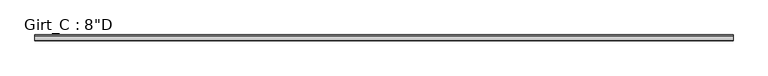
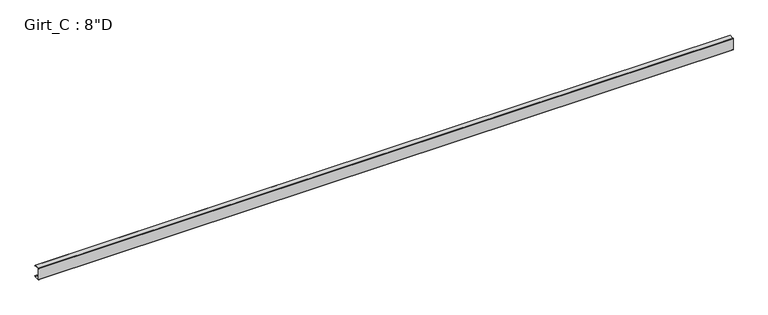
"""IFC4 building model written with IfcOpenShell, lengths in millimetres: beam geometry."""

from ifc_helpers import new_model, si_unit, point, frame, frame_2d, origin, place, context, project, spatial, polyline, circle_curve, trimmed, segment, composite_curve, outline, extrude, source, transform, mapped, element, save


def beam_9130b546(model_context):
    return source(origin(), model_context, "Body", "SweptSolid", [
        extrude(outline(composite_curve([segment(polyline([(87.5109375, 101.6), (99.7560415, 87.0068534), (97.6278742, 85.221109), (86.2154765, 98.821875), (3.3005807, 98.821875)]), True, "CONTINUOUS"), segment(trimmed(circle_curve(frame_2d((3.3741066, 96.8381931)), 1.9850441), [point((3.3005807, 98.821875))], [point((1.3890625, 96.8381931))], True, "CARTESIAN"), True, "CONTINUOUS"), segment(polyline([(1.3890625, 96.8381931), (1.3890625, -96.8389339)]), True, "CONTINUOUS"), segment(trimmed(circle_curve(frame_2d((3.3748024, -96.8389339)), 1.9857399), [point((1.3890625, -96.8389339))], [point((3.2694106, -98.821875))], True, "CARTESIAN"), True, "CONTINUOUS"), segment(polyline([(3.2694106, -98.821875), (86.2154765, -98.821875), (97.6510975, -85.1934327), (99.7792647, -86.979177), (87.5109375, -101.6), (3.3734375, -101.6)]), True, "CONTINUOUS"), segment(trimmed(circle_curve(frame_2d((3.3734375, -96.8375)), 4.7625), [point((3.3734375, -101.6))], [point((-1.3890625, -96.8375))], False, "CARTESIAN"), True, "CONTINUOUS"), segment(polyline([(-1.3890625, -96.8375), (-1.3890625, 96.8375)]), True, "CONTINUOUS"), segment(trimmed(circle_curve(frame_2d((3.3734375, 96.8375)), 4.7625), [point((-1.3890625, 96.8375))], [point((3.3734375, 101.6))], False, "CARTESIAN"), True, "CONTINUOUS"), segment(polyline([(3.3734375, 101.6), (87.5109375, 101.6)]), True, "CONTINUOUS")], self_intersect=False)), frame((-5835.65, 0.0, 0.0), z_axis=(1.0, 0.0, 0.0), x_axis=(0.0, 1.0, 0.0)), (0.0, 0.0, 1.0), 11671.3),
    ])


if __name__ == "__main__":
    model = new_model("IFC4")
    model_context = context("Model", 3, world=origin())
    ifc_project = project(units=[si_unit("LENGTHUNIT", "METRE", prefix="MILLI")], contexts=[model_context])
    site = spatial("IfcSite", under=ifc_project)
    building = spatial("IfcBuilding", under=site)
    placement = place(None, origin())
    beam_shape = beam_9130b546(model_context)
    element("IfcBeam", 1, ObjectType="Girt_C : 8\"D", at=placement, inside=building, context=model_context, shape_type="MappedRepresentation", body=[
        mapped(beam_shape, transform((0.0, 0.0, 0.0), x_axis=(1.0, 0.0, 0.0), y_axis=(0.0, 1.0, 0.0), z_axis=(0.0, 0.0, 1.0))),
    ])
    save(model, "model.ifc")

# Revit data of these elements
# Type "Girt_C : 8\"D"
#   half leg = 0' - 1 3/4"
#   Web_Thickness = 0' - 0 7/64"
#   Length [instance default] = 10' - 0"
#   Leg_1 = 0' - 3 1/2"
#   Height = 0' - 8"
#   Structural Material [instance default] = none
# Element 1 (IfcBeam, "Girt_C : 8\"D")
#   Structural Material = CEE' SECTION (8.0x3.5C - SEE STRUCT. DWGS)
#   Materials on its faces: "CEE' SECTION (8.0x3.5C - SEE STRUCT. DWGS)"
# Materials
#   "CEE' SECTION (8.0x3.5C - SEE STRUCT. DWGS)": class "Metal", colour RGB 137 146 153, transparency 0, Description = "Steel, mill finish", Cost = 0
